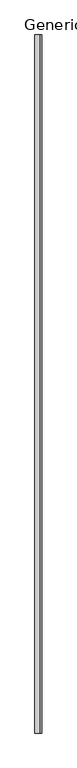
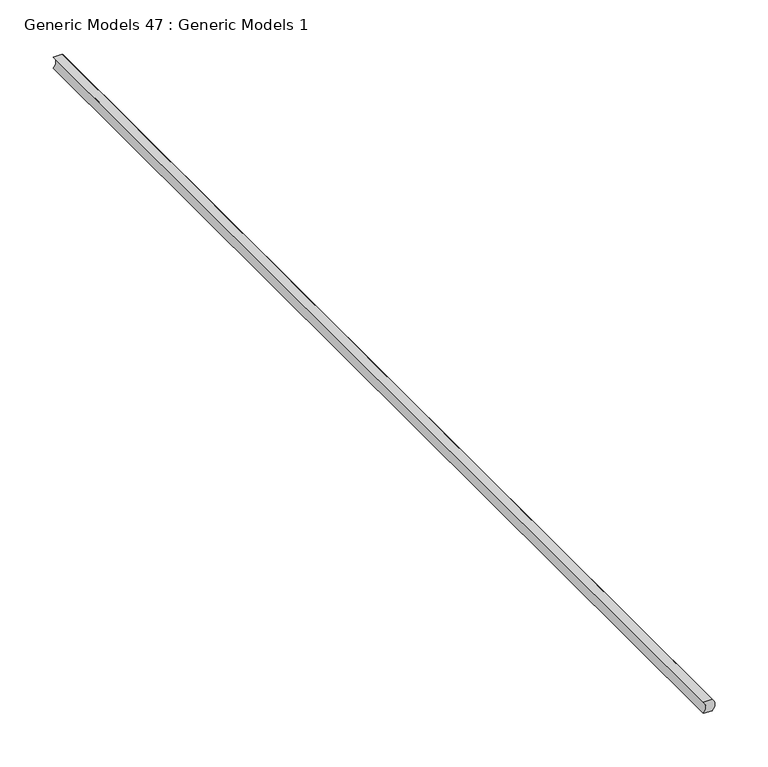
"""IFC4 building model written with IfcOpenShell, lengths in millimetres: proxy geometry, Generic Models 47 : Generic Models 1."""

import ifcopenshell
import ifcopenshell.guid

model = None  # the IFC model being written
_history = None  # IfcOwnerHistory: only IFC2X3 demands one
_inside = {}  # id of a spatial element -> (the spatial element, [elements in it])
_under = {}  # id of a project, library or spatial element -> (it, [spatial elements below it])
_declared = {}  # id of a project -> (the project, [libraries it declares])
_typed = {}  # id of a type object -> (the type object, [elements of that type])
_made_of = {}  # id of a material, layer set ... -> (it, [elements and type objects made of it])


def new_model(schema):
    """Start an empty IFC model of exactly this schema.

    Asked for "IFC4X3", IfcOpenShell would pick the latest addendum, in which some entities
    have other attributes; the version numbers below select the first issue.
    IFC2X3 requires an IfcOwnerHistory on every rooted entity: one is made here for all.
    """
    global model, _history
    if schema == "IFC4X3":
        model = ifcopenshell.file(schema_version=(4, 3, 0, 0))
    else:
        model = ifcopenshell.file(schema=schema)
    _inside.clear()
    _under.clear()
    _declared.clear()
    _typed.clear()
    _made_of.clear()
    _history = None
    if model.schema == "IFC2X3":
        org = make("IfcOrganization", Name="unknown")
        user = make(
            "IfcPersonAndOrganization",
            ThePerson=make("IfcPerson", FamilyName="unknown"),
            TheOrganization=org,
        )
        app = make(
            "IfcApplication",
            ApplicationDeveloper=org,
            Version="unknown",
            ApplicationFullName="unknown",
            ApplicationIdentifier="unknown",
        )
        _history = make(
            "IfcOwnerHistory",
            OwningUser=user,
            OwningApplication=app,
            ChangeAction="ADDED",
            CreationDate=0,
        )
    return model


def make(cls, **values):
    """One entity of the class cls with the attributes given. An attribute that is None is left unset."""
    return model.create_entity(
        cls, **{name: value for name, value in values.items() if value is not None}
    )


def rooted(cls, **values):
    """An entity with a GlobalId (a new one), such as an element, a storey or a relation."""
    return make(cls, GlobalId=ifcopenshell.guid.new(), OwnerHistory=_history, **values)


def si_unit(unit_type, name, prefix=None):
    """IfcSIUnit, for example si_unit("LENGTHUNIT", "METRE", prefix="MILLI")."""
    return make("IfcSIUnit", UnitType=unit_type, Prefix=prefix, Name=name)


def assignment(units):
    """IfcUnitAssignment: the units of a project."""
    return None if units is None else make("IfcUnitAssignment", Units=units)


def point(xyz):
    """IfcCartesianPoint."""
    return None if xyz is None else make("IfcCartesianPoint", Coordinates=xyz)


def direction(xyz):
    """IfcDirection."""
    return None if xyz is None else make("IfcDirection", DirectionRatios=xyz)


def frame(location, z_axis=None, x_axis=None):
    """IfcAxis2Placement3D, a coordinate frame: its origin and axes. An axis left out is left unset."""
    return make(
        "IfcAxis2Placement3D",
        Location=point(location),
        Axis=direction(z_axis),
        RefDirection=direction(x_axis),
    )


def frame_2d(location, x_axis=None):
    """IfcAxis2Placement2D, a coordinate frame in the plane: its origin and x axis."""
    return make(
        "IfcAxis2Placement2D", Location=point(location), RefDirection=direction(x_axis)
    )


def origin():
    """The frame at (0, 0, 0) with its axes left unset."""
    return frame((0.0, 0.0, 0.0))


def place(relative_to, where):
    """IfcLocalPlacement: puts the frame where relative to a parent placement (None: the world)."""
    return make(
        "IfcLocalPlacement", PlacementRelTo=relative_to, RelativePlacement=where
    )


def context(
    kind, dimensions, precision=None, world=None, true_north=None, identifier=None
):
    """IfcGeometricRepresentationContext, for example the 3D "Model" context."""
    return make(
        "IfcGeometricRepresentationContext",
        ContextIdentifier=identifier,
        ContextType=kind,
        CoordinateSpaceDimension=dimensions,
        Precision=precision,
        WorldCoordinateSystem=world,
        TrueNorth=true_north,
    )


def project(units=None, contexts=None):
    """IfcProject with its units and contexts."""
    return rooted(
        "IfcProject",
        Name="project",
        RepresentationContexts=contexts,
        UnitsInContext=assignment(units),
    )


def spatial(cls, under=None, at=None, **own):
    """A site, building, storey or space (cls), placed at a placement, below another one or the project."""
    s = rooted(cls, ObjectPlacement=at, **own)
    if under is not None:
        _under.setdefault(under.id(), (under, []))[1].append(s)
    return s


def polyline(points):
    """IfcPolyline through the points."""
    return make("IfcPolyline", Points=[point(p) for p in points])


def circle_curve(where, radius):
    """IfcCircle in the frame where."""
    return make("IfcCircle", Position=where, Radius=radius)


def trimmed(basis, trim1, trim2, sense, master):
    """IfcTrimmedCurve: the piece of a basis curve between two trims."""
    return make(
        "IfcTrimmedCurve",
        BasisCurve=basis,
        Trim1=trim1,
        Trim2=trim2,
        SenseAgreement=sense,
        MasterRepresentation=master,
    )


def segment(curve, same_sense, transition):
    """IfcCompositeCurveSegment."""
    return make(
        "IfcCompositeCurveSegment",
        Transition=transition,
        SameSense=same_sense,
        ParentCurve=curve,
    )


def composite_curve(segments, self_intersect=None):
    """IfcCompositeCurve: segments joined end to end."""
    return make("IfcCompositeCurve", Segments=segments, SelfIntersect=self_intersect)


def outline(outer, holes=None, kind="AREA"):
    """IfcArbitraryClosedProfileDef: a profile drawn as a closed curve; with holes, ...WithVoids."""
    if holes is None:
        return make("IfcArbitraryClosedProfileDef", ProfileType=kind, OuterCurve=outer)
    return make(
        "IfcArbitraryProfileDefWithVoids",
        ProfileType=kind,
        OuterCurve=outer,
        InnerCurves=holes,
    )


def extrude(swept, where, along, depth):
    """IfcExtrudedAreaSolid: the profile swept, set in the frame where, extruded along a direction by depth."""
    return make(
        "IfcExtrudedAreaSolid",
        SweptArea=swept,
        Position=where,
        ExtrudedDirection=direction(along),
        Depth=depth,
    )


def shape(context_of_items, identifier, shape_type, items):
    """IfcShapeRepresentation: the items that make up one representation, for example the "Body"."""
    return make(
        "IfcShapeRepresentation",
        ContextOfItems=context_of_items,
        RepresentationIdentifier=identifier,
        RepresentationType=shape_type,
        Items=items,
    )


def source(mapping_origin, context_of_items, identifier, shape_type, items):
    """IfcRepresentationMap: a shape defined once, which mapped items show again and again."""
    return make(
        "IfcRepresentationMap",
        MappingOrigin=mapping_origin,
        MappedRepresentation=shape(context_of_items, identifier, shape_type, items),
    )


def transform(
    local_origin,
    x_axis=None,
    y_axis=None,
    z_axis=None,
    scale=None,
    scale2=None,
    scale3=None,
    uniform=True,
):
    """IfcCartesianTransformationOperator3D, or its non-uniform kind. x_axis, y_axis, z_axis: its Axis1, 2, 3."""
    if uniform:
        return make(
            "IfcCartesianTransformationOperator3D",
            Axis1=direction(x_axis),
            Axis2=direction(y_axis),
            LocalOrigin=point(local_origin),
            Scale=scale,
            Axis3=direction(z_axis),
        )
    return make(
        "IfcCartesianTransformationOperator3DnonUniform",
        Axis1=direction(x_axis),
        Axis2=direction(y_axis),
        LocalOrigin=point(local_origin),
        Scale=scale,
        Axis3=direction(z_axis),
        Scale2=scale2,
        Scale3=scale3,
    )


def mapped(mapping_source, mapping_target):
    """IfcMappedItem: shows the shape of a source again, moved by a transform."""
    return make(
        "IfcMappedItem", MappingSource=mapping_source, MappingTarget=mapping_target
    )


def made_of(thing, what):
    """Note that an element or type object is made of a material, layer set ...; save() writes the relation."""
    if what is not None:
        _made_of.setdefault(what.id(), (what, []))[1].append(thing)
    return thing


def element(
    cls,
    number,
    at=None,
    inside=None,
    cuts=None,
    type_object=None,
    material=None,
    context=None,
    identifier="Body",
    shape_type=None,
    held_by="IfcProductDefinitionShape",
    body=None,
    shapes=None,
    **own,
):
    """One element of the class cls, such as IfcWall. Its Tag is "e" and its number.

    at: its placement. inside: the storey or other place that contains it. cuts: it is an
    opening in that element (IfcRelVoidsElement). A single representation is given by context,
    identifier, shape_type and body (its items); several are given by shapes. held_by: the class
    of the entity that holds the representations. save() writes the other relations.
    """
    e = rooted(cls, Tag="e%d" % number, ObjectPlacement=at, **own)
    if body is not None:
        shapes = [shape(context, identifier, shape_type, body)]
    if shapes is not None:
        e.Representation = make(held_by, Representations=shapes)
    if inside is not None:
        _inside.setdefault(inside.id(), (inside, []))[1].append(e)
    if cuts is not None:
        rooted(
            "IfcRelVoidsElement", RelatingBuildingElement=cuts, RelatedOpeningElement=e
        )
    if type_object is not None:
        _typed.setdefault(type_object.id(), (type_object, []))[1].append(e)
    return made_of(e, material)


def aggregate(whole, parts):
    """IfcRelAggregates: a whole, such as a stair, and the parts it consists of."""
    return rooted("IfcRelAggregates", RelatingObject=whole, RelatedObjects=parts)


def save(model, path):
    """Write the relations noted so far, then the file.

    IfcRelAggregates (storeys below a building ...), IfcRelContainedInSpatialStructure (elements
    in a storey), IfcRelDefinesByType, IfcRelAssociatesMaterial and IfcRelDeclares: one each for
    every whole, place, type object, material and project.
    """
    for whole, parts in _under.values():
        aggregate(whole, parts)
    for where, things in _inside.values():
        rooted(
            "IfcRelContainedInSpatialStructure",
            RelatedElements=things,
            RelatingStructure=where,
        )
    for kind, things in _typed.values():
        rooted("IfcRelDefinesByType", RelatedObjects=things, RelatingType=kind)
    for what, things in _made_of.values():
        rooted("IfcRelAssociatesMaterial", RelatedObjects=things, RelatingMaterial=what)
    for by, libraries in _declared.values():
        rooted("IfcRelDeclares", RelatingContext=by, RelatedDefinitions=libraries)
    model.write(path)


def generic_models_47_generic_models_1_9e68d635(model_context):
    return source(origin(), model_context, "Body", "SweptSolid", [
        extrude(outline(composite_curve([segment(polyline([(2438.4, 50759.2377541), (2438.4, 50768.7627541)]), True, "CONTINUOUS"), segment(trimmed(circle_curve(frame_2d((2444.75, 50762.9332731)), 8.620055), [point((2438.4, 50768.7627541))], [point((2451.1, 50768.7627541))], False, "CARTESIAN"), True, "CONTINUOUS"), segment(polyline([(2451.1, 50768.7627541), (2451.1, 50759.2377541)]), True, "CONTINUOUS"), segment(trimmed(circle_curve(frame_2d((2444.75, 50753.4082731)), 8.620055), [point((2451.1, 50759.2377541))], [point((2438.4, 50759.2377541))], True, "CARTESIAN"), True, "CONTINUOUS")], self_intersect=False)), frame((0.0, 0.0, 0.0), z_axis=(0.0, 1.0, 0.0), x_axis=(0.0, 0.0, 1.0)), (0.0, 0.0, 1.0), 1219.2),
    ])


if __name__ == "__main__":
    model = new_model("IFC4")
    model_context = context("Model", 3, world=origin())
    ifc_project = project(units=[si_unit("LENGTHUNIT", "METRE", prefix="MILLI")], contexts=[model_context])
    site = spatial("IfcSite", under=ifc_project)
    building = spatial("IfcBuilding", under=site)
    placement = place(None, origin())
    generic_models_47_generic_models_1_shape = generic_models_47_generic_models_1_9e68d635(model_context)
    element("IfcBuildingElementProxy", 1, Name="Generic Models 47 : Generic Models 1", ObjectType="Generic Models 47 : Generic Models 1", at=placement, inside=building, context=model_context, shape_type="MappedRepresentation", body=[
        mapped(generic_models_47_generic_models_1_shape, transform((0.0, 0.0, 0.0), x_axis=(1.0, 0.0, 0.0), y_axis=(0.0, 1.0, 0.0), z_axis=(0.0, 0.0, 1.0))),
    ])
    save(model, "model.ifc")

# Revit data of these elements
# Element 1 (IfcBuildingElementProxy, "Generic Models 47 : Generic Models 1")
#   Materials on its faces: "ACOUSTICAL SEALANT"
# Materials
#   "ACOUSTICAL SEALANT": class "Unassigned", colour RGB 120 120 120, transparency 0, Cost = 0
